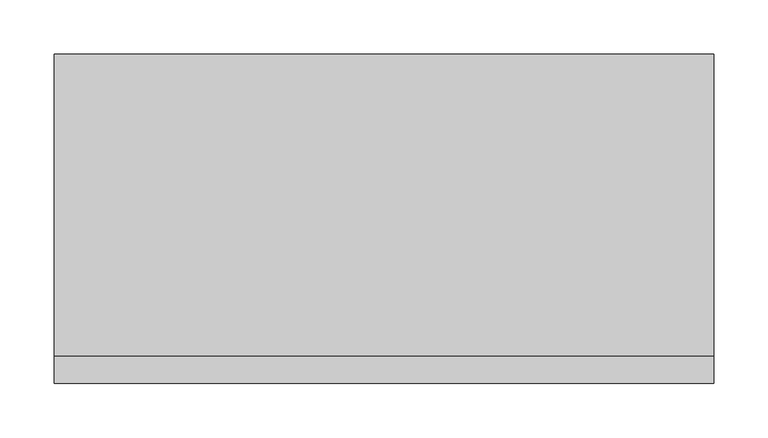
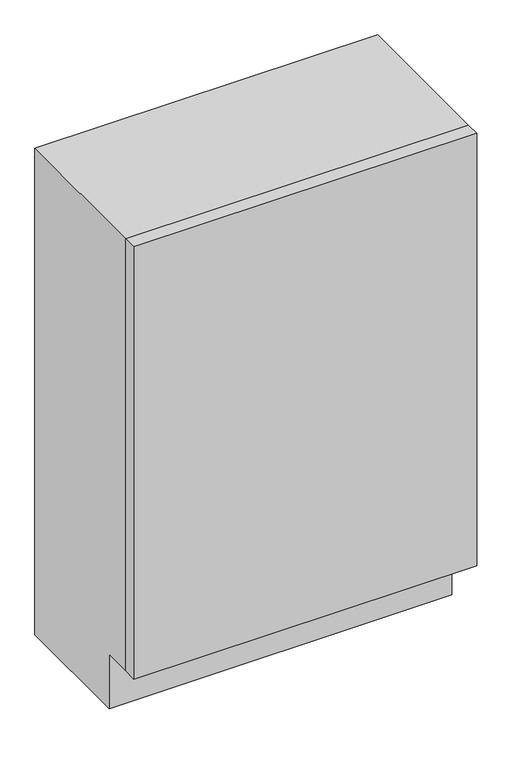
"""IFC4 building model written with IfcOpenShell, lengths in millimetres: furniture geometry, OD_CW_Base Cabinet : OD_CW_Base Cabinet."""

from ifc_helpers import new_model, si_unit, frame, origin, place, context, project, spatial, polyline, outline, extrude, source, transform, mapped, element, save


def furniture_f3df3c95(model_context):
    return source(origin(), model_context, "Body", "SweptSolid", [
        extrude(outline(polyline([(18.7377049, 330.2), (628.3377049, 330.2), (628.3377049, 304.8), (18.7377049, 304.8), (18.7377049, 330.2)])), frame((0.0, 0.0, 101.6), z_axis=(0.0, 0.0, 1.0), x_axis=(1.0, 0.0, 0.0)), (0.0, 0.0, 1.0), 812.8),
        extrude(outline(polyline([(330.2, 914.4), (609.6, 914.4), (609.6, 0.0), (381.0, 0.0), (381.0, 101.6), (330.2, 101.6), (330.2, 914.4)])), frame((18.7377049, 0.0, 0.0), z_axis=(1.0, 0.0, 0.0), x_axis=(0.0, 1.0, 0.0)), (0.0, 0.0, 1.0), 609.6),
    ])


if __name__ == "__main__":
    model = new_model("IFC4")
    model_context = context("Model", 3, world=origin())
    ifc_project = project(units=[si_unit("LENGTHUNIT", "METRE", prefix="MILLI")], contexts=[model_context])
    site = spatial("IfcSite", under=ifc_project)
    building = spatial("IfcBuilding", under=site)
    placement = place(None, origin())
    furniture_shape = furniture_f3df3c95(model_context)
    element("IfcFurniture", 1, ObjectType="OD_CW_Base Cabinet : OD_CW_Base Cabinet", at=placement, inside=building, context=model_context, shape_type="MappedRepresentation", body=[
        mapped(furniture_shape, transform((0.0, 0.0, 0.0), x_axis=(1.0, 0.0, 0.0), y_axis=(0.0, 1.0, 0.0), z_axis=(0.0, 0.0, 1.0))),
    ])
    save(model, "model.ifc")

# Revit data of these elements
# Type "OD_CW_Base Cabinet : OD_CW_Base Cabinet"
#   OD_CW_Width [instance default] = 2' - 10"
#   OD_CW_Length [instance default] = 8' - 0"
#   OD_CW_Height [instance default] = 2' - 3"
#   Depth = 2' - 0"
#   Height = 3' - 0"
#   Width = 4' - 0"
#   OD_CW_Material_Front Panel [instance default] = none
#   OD_CW_Material_Body [instance default] = none
# Element 1 (IfcFurniture, "OD_CW_Base Cabinet : OD_CW_Base Cabinet")
#   OD_CW_Width = 1' - 0"
#   OD_CW_Length = 2' - 0"
#   OD_CW_Height = 3' - 0"
#   OD_CW_Material_Body = HW SINK
#   Materials on its faces: "HW SINK", "CASEWORK"
# Materials
#   "HW SINK": class "Generic", colour RGB 187 187 187, transparency 0, Cost = 0
#   "CASEWORK": class "Generic", colour RGB 181 181 181, transparency 0, Cost = 0
